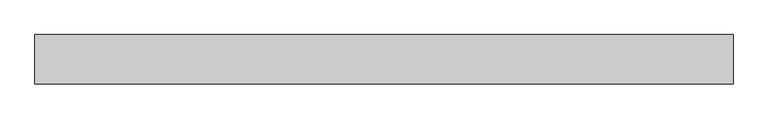
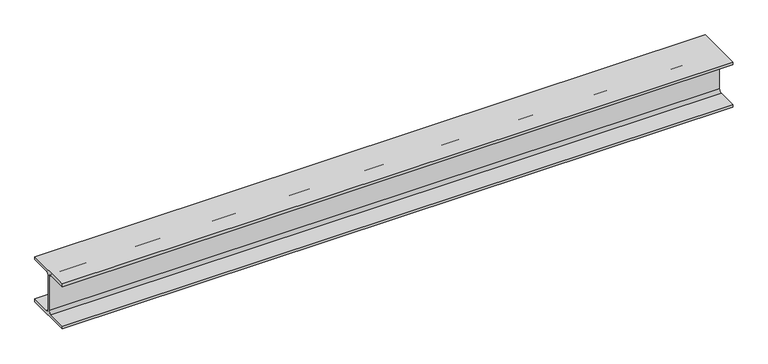
"""IFC4 building model written with IfcOpenShell, lengths in millimetres: beam geometry, 0912_Steel Framing_H-KSD3502 : H_SB_ASB_H-200x200x8x12."""

from ifc_helpers import new_model, si_unit, point, frame, frame_2d, origin, place, context, project, spatial, polyline, circle_curve, trimmed, segment, composite_curve, outline, extrude, source, transform, mapped, element, save


def beam_015ba6da(model_context):
    return source(origin(), model_context, "Body", "SweptSolid", [
        extrude(outline(composite_curve([segment(polyline([(100.0, -88.0), (100.0, -100.0), (-100.0, -100.0), (-100.0, -88.0), (-17.0, -88.0)]), True, "CONTINUOUS"), segment(trimmed(circle_curve(frame_2d((-17.0, -75.0)), 13.0), [point((-17.0, -88.0))], [point((-4.0, -75.0))], True, "CARTESIAN"), True, "CONTINUOUS"), segment(polyline([(-4.0, -75.0), (-4.0, 75.0)]), True, "CONTINUOUS"), segment(trimmed(circle_curve(frame_2d((-17.0, 75.0)), 13.0), [point((-4.0, 75.0))], [point((-17.0, 88.0))], True, "CARTESIAN"), True, "CONTINUOUS"), segment(polyline([(-17.0, 88.0), (-100.0, 88.0), (-100.0, 100.0), (100.0, 100.0), (100.0, 88.0), (17.0, 88.0)]), True, "CONTINUOUS"), segment(trimmed(circle_curve(frame_2d((17.0, 75.0)), 13.0), [point((17.0, 88.0))], [point((4.0, 75.0))], True, "CARTESIAN"), True, "CONTINUOUS"), segment(polyline([(4.0, 75.0), (4.0, -75.0)]), True, "CONTINUOUS"), segment(trimmed(circle_curve(frame_2d((17.0, -75.0)), 13.0), [point((4.0, -75.0))], [point((17.0, -88.0))], True, "CARTESIAN"), True, "CONTINUOUS"), segment(polyline([(17.0, -88.0), (100.0, -88.0)]), True, "CONTINUOUS")], self_intersect=False)), frame((-1249.4797233, 0.0, 0.0), z_axis=(1.0, 0.0, 0.0), x_axis=(0.0, 1.0, 0.0)), (0.0, 0.0, 1.0), 2817.4800203),
    ])


if __name__ == "__main__":
    model = new_model("IFC4")
    model_context = context("Model", 3, world=origin())
    ifc_project = project(units=[si_unit("LENGTHUNIT", "METRE", prefix="MILLI")], contexts=[model_context])
    site = spatial("IfcSite", under=ifc_project)
    building = spatial("IfcBuilding", under=site)
    placement = place(None, origin())
    beam_shape = beam_015ba6da(model_context)
    element("IfcBeam", 1, ObjectType="0912_Steel Framing_H-KSD3502 : H_SB_ASB_H-200x200x8x12", at=placement, inside=building, context=model_context, shape_type="MappedRepresentation", body=[
        mapped(beam_shape, transform((0.0, 0.0, 0.0), x_axis=(1.0, 0.0, 0.0), y_axis=(0.0, 1.0, 0.0), z_axis=(0.0, 0.0, 1.0))),
    ])
    save(model, "model.ifc")

# Revit data of these elements
# Type "0912_Steel Framing_H-KSD3502 : H_SB_ASB_H-200x200x8x12"
#   H_WM Code_1 = "S01AA002-00001 | Main Steel Structure Fabrication Work | Shelter/Building | Medium Steel - Standard (90KG/M>Weight≥30KG/M) | Material: (   )"
#   H_WM Code_2 = "S03AA028-00001 | Main Steel Structure Erection Work | Shelter/Building | Medium Steel (90KG/M>Weight≥30KG/M) | Material: (   )"
#   H_WM Code_3 = "S01AA010-00001 | Main Steel Structure Fabrication Work | Shelter/Building | Steel Painting/Coating | for Non-Fireproofed Steel Surface, Surface Preparation, Primer, Second & Final Coat | Material: (   )"
#   H_Q'ty Cal Type Tag = "SB-Q2"
#   Width = 20.0 cm
#   Web Thickness = 0.8 cm
#   Web Fillet = 1.3 cm
#   Warping Constant = 141000.0 cm⁶
#   W = 0
#   Torsional Moment of Inertia = 26.2485 cm⁴
#   Section Area = 63.53 cm²
#   Plastic Modulus weak axis = 244.0 cm³
#   Plastic Modulus strong axis = 525.0 cm³
#   Perimeter = 1.16 m²/m
#   Nominal Weight = 49.90 kgf/m
#   Moment of Inertia weak axis = 1600.00 cm⁴
#   Moment of Inertia strong axis = 4720.00 cm⁴
#   Height = 20.0 cm
#   Flange Thickness = 1.2 cm
#   Elastic Modulus weak axis = 160.0 cm³
#   Elastic Modulus strong axis = 472.0 cm³
#   Centroid Vertical = 10.0 cm
#   Centroid Horizontal = 10.0 cm
#   Ix = 47200000
#   Length [instance default] = 1.5240 m
#   Zx = 525000
#   b = 0.2000 m
#   h = 0.2000 m
#   r = 0.0130 m
#   s = 0.0080 m
#   t = 0.0120 m
#   A = 0.006353 m²
#   Structural Material [instance default] = Steel, 45-345
#   Assembly Code = ""
# Element 1 (IfcBeam, "0912_Steel Framing_H-KSD3502 : H_SB_ASB_H-200x200x8x12")
#   Structural Material = none
# Materials
#   "Steel, 45-345": class "Metal", colour RGB 189 187 185, transparency 0, Description = "Steel 345 MPa", Cost = 0
